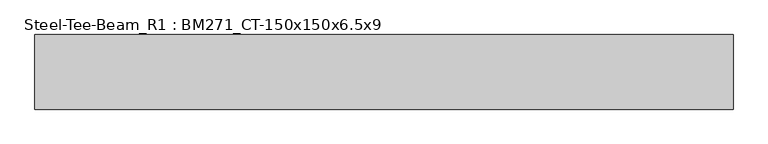
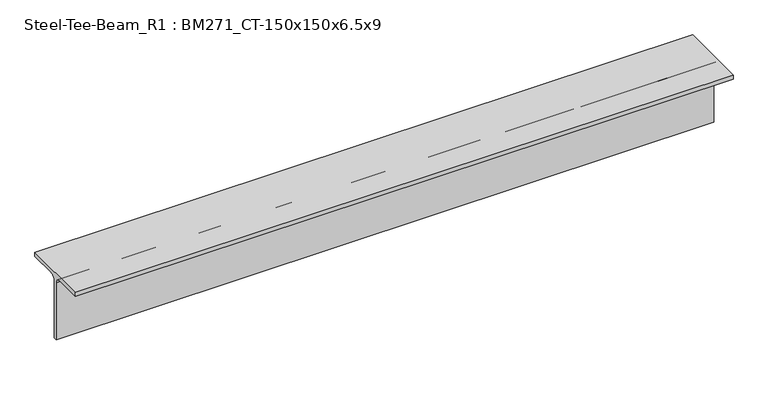
"""IFC4 building model written with IfcOpenShell, lengths in millimetres: member geometry, Steel-Tee-Beam_R1 : BM271_CT-150x150x6.5x9."""

from ifc_helpers import new_model, si_unit, point, frame, frame_2d, origin, place, context, project, spatial, polyline, circle_curve, trimmed, segment, composite_curve, outline, extrude, source, transform, mapped, element, save


def steel_tee_beam_r1_bm271_ct_150x150x6_5x9_1fc16235(model_context):
    return source(origin(), model_context, "Body", "SweptSolid", [
        extrude(outline(composite_curve([segment(polyline([(75.0, 75.0), (75.0, 66.0), (16.25, 66.0)]), True, "CONTINUOUS"), segment(trimmed(circle_curve(frame_2d((16.25, 53.0)), 13.0), [point((16.25, 66.0))], [point((3.25, 53.0))], True, "CARTESIAN"), True, "CONTINUOUS"), segment(polyline([(3.25, 53.0), (3.25, -75.0), (-3.25, -75.0), (-3.25, 53.0)]), True, "CONTINUOUS"), segment(trimmed(circle_curve(frame_2d((-16.25, 53.0)), 13.0), [point((-3.25, 53.0))], [point((-16.25, 66.0))], True, "CARTESIAN"), True, "CONTINUOUS"), segment(polyline([(-16.25, 66.0), (-75.0, 66.0), (-75.0, 75.0), (75.0, 75.0)]), True, "CONTINUOUS")], self_intersect=False)), frame((-701.7933274, 0.0, 0.0), z_axis=(1.0, 0.0, 0.0), x_axis=(0.0, 1.0, 0.0)), (0.0, 0.0, 1.0), 1403.5866548),
    ])


if __name__ == "__main__":
    model = new_model("IFC4")
    model_context = context("Model", 3, world=origin())
    ifc_project = project(units=[si_unit("LENGTHUNIT", "METRE", prefix="MILLI")], contexts=[model_context])
    site = spatial("IfcSite", under=ifc_project)
    building = spatial("IfcBuilding", under=site)
    placement = place(None, origin())
    steel_tee_beam_r1_bm271_ct_150x150x6_5x9_shape = steel_tee_beam_r1_bm271_ct_150x150x6_5x9_1fc16235(model_context)
    element("IfcMember", 1, ObjectType="Steel-Tee-Beam_R1 : BM271_CT-150x150x6.5x9", at=placement, inside=building, context=model_context, shape_type="MappedRepresentation", body=[
        mapped(steel_tee_beam_r1_bm271_ct_150x150x6_5x9_shape, transform((0.0, 0.0, 0.0), x_axis=(1.0, 0.0, 0.0), y_axis=(0.0, 1.0, 0.0), z_axis=(0.0, 0.0, 1.0))),
    ])
    save(model, "model.ifc")

# Revit data of these elements
# Type "Steel-Tee-Beam_R1 : BM271_CT-150x150x6.5x9"
#   Keynote = "CT-150x150x6.5x9"
#   Surface Area = 0.588841 m²/m
#   Section Area = 23.3904 cm²
#   Mass per Unit Length = 18.3614 kg/m
#   Length [instance default] = 1.5240 m
#   bf = 0.1500 m
#   d = 0.1500 m
#   k = 0.0220 m
#   r = 0.0130 m
#   tf = 0.0090 m
#   tw = 0.0065 m
#   hec_material4 [instance default] = none
#   hec_material3 [instance default] = none
#   hec_material2 [instance default] = none
#   hec_material1 [instance default] = none
#   Structural Material [instance default] = Steel, 45-345
#   Assembly Code = ""
# Element 1 (IfcMember, "Steel-Tee-Beam_R1 : BM271_CT-150x150x6.5x9")
#   Structural Material = none
# Materials
#   "Steel, 45-345": class "Metal", colour RGB 189 187 185, transparency 0, Description = "Steel 345 MPa", Cost = 0
